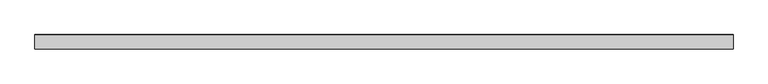
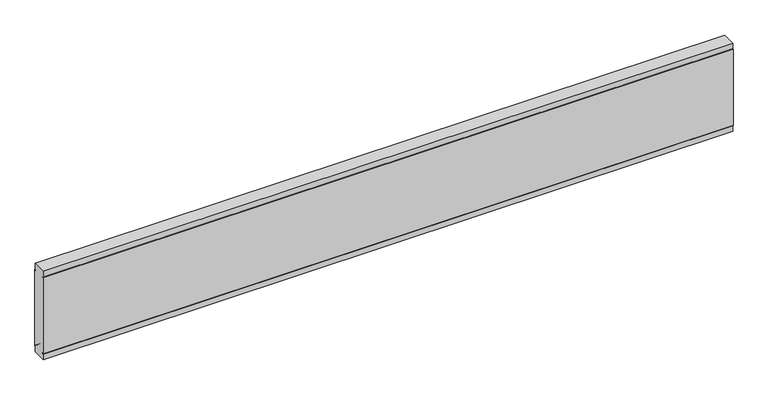
"""IFC4 building model written with IfcOpenShell, lengths in millimetres: proxy geometry, Generic Models 7:Generic Models 1:5:Generic Models 1:5 : Generic Models 7:Generic Models 1:337419:8 : Generic Models 7:Generic Models 1:5:Generic Models 1:5 : Generic Models 7:Generic Models 1:337419:311462."""

from ifc_helpers import new_model, si_unit, frame, origin, place, context, project, spatial, polyline, outline, extrude, source, transform, mapped, element, save


def generic_models_25e68b50(model_context):
    return source(origin(), model_context, "Body", "SweptSolid", [
        extrude(outline(polyline([(-578799.0788841, 4893.9308169), (-578799.0788841, 3767.0723081), (-578812.2802009, 3778.1495282), (-578816.1067959, 3773.5891699), (-578801.8570091, 3761.632179), (-578801.8570091, 3679.428125), (-578996.3257591, 3679.428125), (-578996.3257591, 3761.632179), (-578982.0759722, 3773.5891699), (-578985.9025672, 3778.1495282), (-578999.1038841, 3767.0723081), (-578999.1038841, 4893.9308169), (-578985.9025672, 4882.8535968), (-578982.0759722, 4887.4139551), (-578996.3257591, 4899.370946), (-578996.3257591, 4981.575), (-578801.8570091, 4981.575), (-578801.8570091, 4899.370946), (-578816.1067959, 4887.4139551), (-578812.2802009, 4882.8535968), (-578799.0788841, 4893.9308169)])), frame((560859.6126799, 0.0, 0.0), z_axis=(1.0, 0.0, 0.0), x_axis=(0.0, 1.0, 0.0)), (0.0, 0.0, 1.0), 9631.124044),
    ])


if __name__ == "__main__":
    model = new_model("IFC4")
    model_context = context("Model", 3, world=origin())
    ifc_project = project(units=[si_unit("LENGTHUNIT", "METRE", prefix="MILLI")], contexts=[model_context])
    site = spatial("IfcSite", under=ifc_project)
    building = spatial("IfcBuilding", under=site)
    placement = place(None, origin())
    generic_models_shape = generic_models_25e68b50(model_context)
    element("IfcBuildingElementProxy", 1, Name="Generic Models 7:Generic Models 1:5:Generic Models 1:5 : Generic Models 7:Generic Models 1:337419:8 : Generic Models 7:Generic Models 1:5:Generic Models 1:5 : Generic Models 7:Generic Models 1:337419:311462", ObjectType="Generic Models 7:Generic Models 1:5:Generic Models 1:5 : Generic Models 7:Generic Models 1:337419:8 : Generic Models 7:Generic Models 1:5:Generic Models 1:5 : Generic Models 7:Generic Models 1:337419:311462", at=placement, inside=building, context=model_context, shape_type="MappedRepresentation", body=[
        mapped(generic_models_shape, transform((0.0, 0.0, 0.0), x_axis=(1.0, 0.0, 0.0), y_axis=(0.0, 1.0, 0.0), z_axis=(0.0, 0.0, 1.0))),
    ])
    save(model, "model.ifc")

# Revit data of these elements
# Type "Generic Models 7:Generic Models 1:5:Generic Models 1:5 : Generic Models 7:Generic Models 1:337419:8 : Generic Models 7:Generic Models 1:5:Generic Models 1:5 : Generic Models 7:Generic Models 1:337419:311462"
#   NameOverride = "Generic Models 7:Generic Models 1:5:Generic Models 1:5 : Generic Models 7:Generic Models 1:337419:311462"
#   ObjectTypeOverride = "Generic Models 1:5 : Generic Models 7:Generic Models 1:337419"
#   Reference = "Generic Models 1"
#   Tag = "311462"
# Element 1 (IfcBuildingElementProxy, "Generic Models 7:Generic Models 1:5:Generic Models 1:5 : Generic Models 7:Generic Models 1:337419:8 : Generic Models 7:Generic Models 1:5:Generic Models 1:5 : Generic Models 7:Generic Models 1:337419:311462")
#   Materials on its faces: "SIMPLE SAVER INSULATION WITH LINER - COLOR: BLACK"
# Materials
#   "SIMPLE SAVER INSULATION WITH LINER - COLOR: BLACK": class "Unassigned", colour RGB 158 92 175, transparency 0, Cost = 0
